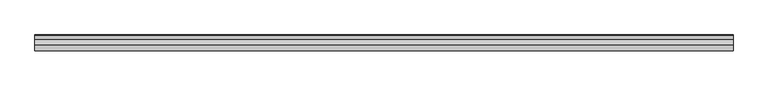
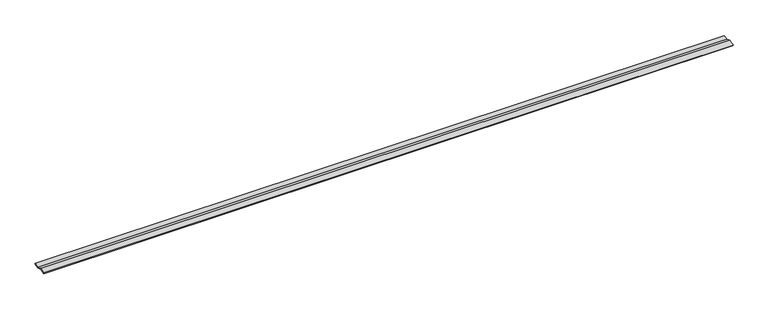
"""IFC4 building model written with IfcOpenShell, lengths in millimetres: proxy geometry, Gutter @ Roof004 35472 : Gutter @ Roof004 35472."""

from ifc_helpers import new_model, si_unit, frame, origin, place, context, project, spatial, polyline, outline, extrude, source, transform, mapped, element, save


def generic_models_2a12b37d(model_context):
    return source(origin(), model_context, "Body", "SweptSolid", [
        extrude(outline(polyline([(-5227.7746422, 42846.6894729), (-5213.6083006, 42841.7188154), (-5200.2540881, 42845.1047805), (-5199.629824, 42842.6426891), (-5213.726504, 42839.0684711), (-5227.8868147, 42844.0370125), (-5243.936465, 42839.8887832), (-5244.5720722, 42842.3479707), (-5227.7746422, 42846.6894729)])), frame((12382.7678845, 0.0, 0.0), z_axis=(1.0, 0.0, 0.0), x_axis=(0.0, 1.0, 0.0)), (0.0, 0.0, 1.0), 2000.25),
    ])


if __name__ == "__main__":
    model = new_model("IFC4")
    model_context = context("Model", 3, world=origin())
    ifc_project = project(units=[si_unit("LENGTHUNIT", "METRE", prefix="MILLI")], contexts=[model_context])
    site = spatial("IfcSite", under=ifc_project)
    building = spatial("IfcBuilding", under=site)
    placement = place(None, origin())
    generic_models_shape = generic_models_2a12b37d(model_context)
    element("IfcBuildingElementProxy", 1, Name="Gutter @ Roof004 35472 : Gutter @ Roof004 35472", ObjectType="Gutter @ Roof004 35472 : Gutter @ Roof004 35472", at=placement, inside=building, context=model_context, shape_type="MappedRepresentation", body=[
        mapped(generic_models_shape, transform((0.0, 0.0, 0.0), x_axis=(1.0, 0.0, 0.0), y_axis=(0.0, 1.0, 0.0), z_axis=(0.0, 0.0, 1.0))),
    ])
    save(model, "model.ifc")

# Revit data of these elements
# Type "Gutter @ Roof004 35472 : Gutter @ Roof004 35472"
#   NameOverride = "Gutter @ Roof004"
# Element 1 (IfcBuildingElementProxy, "Gutter @ Roof004 35472 : Gutter @ Roof004 35472")
#   Materials on its faces: "CONT. SEAMLESS 16 GA COPPER BRAKE METAL GUTTER"
# Materials
#   "CONT. SEAMLESS 16 GA COPPER BRAKE METAL GUTTER": class "Unassigned", colour RGB 128 128 128, transparency 0
